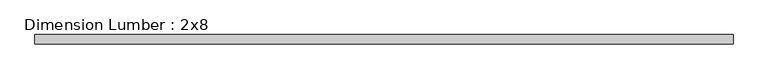
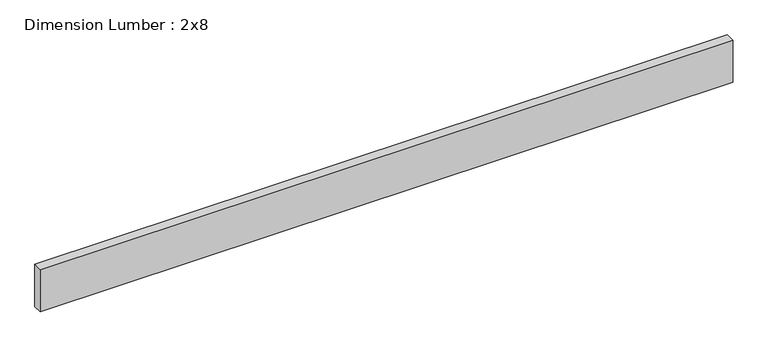
"""IFC4 building model written with IfcOpenShell, lengths in millimetres: beam geometry, Dimension Lumber : 2x8."""

from ifc_helpers import new_model, si_unit, frame, origin, place, context, project, spatial, polyline, outline, extrude, source, transform, mapped, element, save


def dimension_lumber_2x8_d6280bfe(model_context):
    return source(origin(), model_context, "Body", "SweptSolid", [
        extrude(outline(polyline([(2227.6894756, -19.05), (-635.0311633, -19.05), (-635.0311633, 19.05), (2227.6894756, 19.05), (2227.6894756, -19.05)])), frame((0.0, 0.0, -92.075), z_axis=(0.0, 0.0, 1.0), x_axis=(1.0, 0.0, 0.0)), (0.0, 0.0, 1.0), 184.15),
    ])


if __name__ == "__main__":
    model = new_model("IFC4")
    model_context = context("Model", 3, world=origin())
    ifc_project = project(units=[si_unit("LENGTHUNIT", "METRE", prefix="MILLI")], contexts=[model_context])
    site = spatial("IfcSite", under=ifc_project)
    building = spatial("IfcBuilding", under=site)
    placement = place(None, origin())
    dimension_lumber_2x8_shape = dimension_lumber_2x8_d6280bfe(model_context)
    element("IfcBeam", 1, ObjectType="Dimension Lumber : 2x8", at=placement, inside=building, context=model_context, shape_type="MappedRepresentation", body=[
        mapped(dimension_lumber_2x8_shape, transform((0.0, 0.0, 0.0), x_axis=(1.0, 0.0, 0.0), y_axis=(0.0, 1.0, 0.0), z_axis=(0.0, 0.0, 1.0))),
    ])
    save(model, "model.ifc")

# Revit data of these elements
# Type "Dimension Lumber : 2x8"
#   Assembly Code = "B10"
#   A = 0.0755556 SF
#   Length [instance default] = 5' - 0"
#   b = 0' - 1 1/2"
#   d = 0' - 7 1/4"
#   Structural Material [instance default] = PRE-ENGINEERED TRUSS @ 24" O.C.
# Element 1 (IfcBeam, "Dimension Lumber : 2x8")
#   Structural Material = 2 X 8 FIELD FRAMED PURLINS
#   Materials on its faces: "2 X 8 FIELD FRAMED PURLINS"
# Materials
#   "PRE-ENGINEERED TRUSS @ 24\" O.C.": class "Wood", colour RGB 255 255 255, transparency 0, Description = "Pinus Echinata", Cost = 0
#   "2 X 8 FIELD FRAMED PURLINS": class "Wood", colour RGB 234 198 147, transparency 0, Description = "Pinus Echinata", Cost = 0
